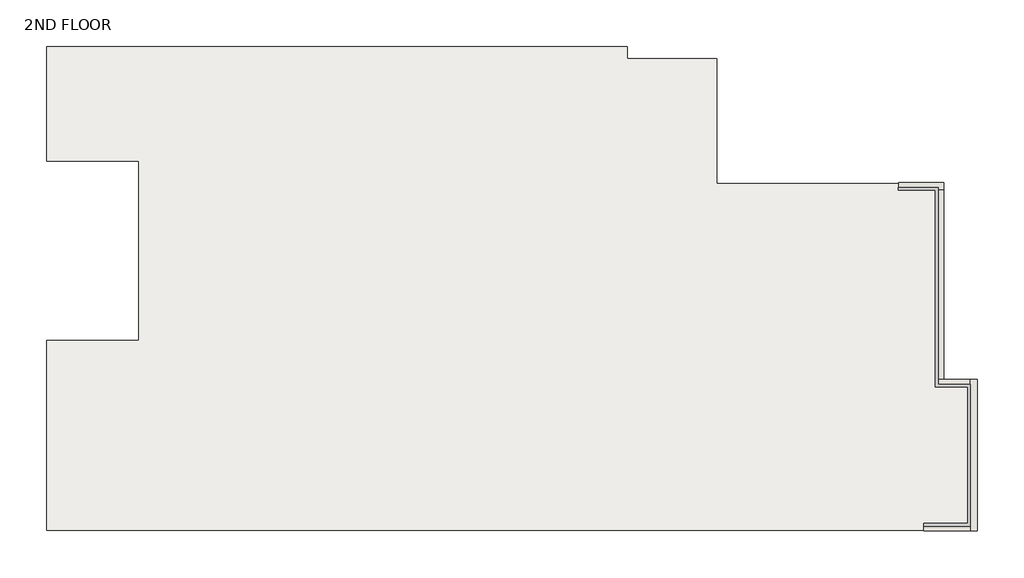
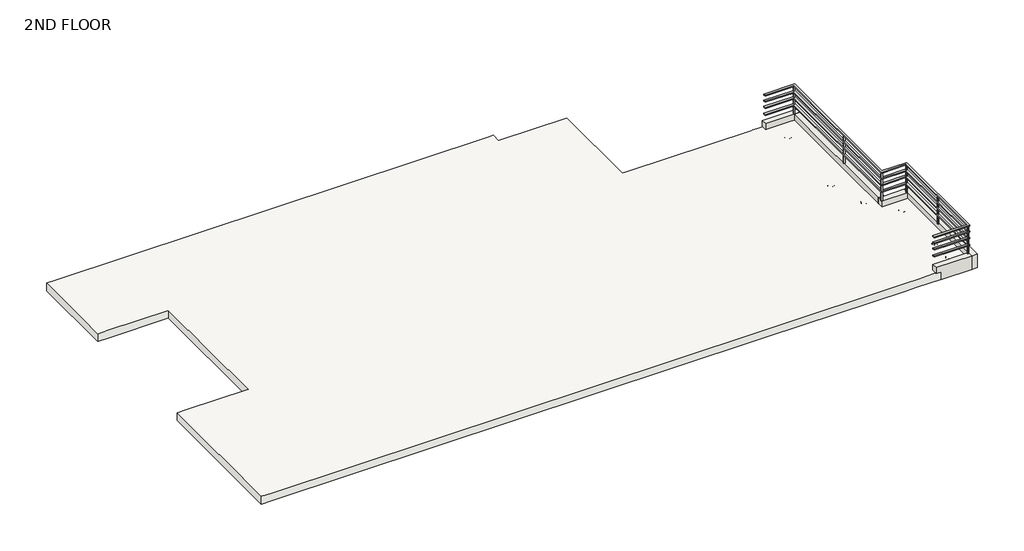
# One storey: 6 geographic elements, 5 proxies, 5 walls, 1 slab.
"""IFC4 building model written with IfcOpenShell, lengths in millimetres."""

import ifcopenshell
import ifcopenshell.guid

model = None  # the IFC model being written
_history = None  # IfcOwnerHistory: only IFC2X3 demands one
_inside = {}  # id of a spatial element -> (the spatial element, [elements in it])
_under = {}  # id of a project, library or spatial element -> (it, [spatial elements below it])
_declared = {}  # id of a project -> (the project, [libraries it declares])
_typed = {}  # id of a type object -> (the type object, [elements of that type])
_made_of = {}  # id of a material, layer set ... -> (it, [elements and type objects made of it])


def new_model(schema):
    """Start an empty IFC model of exactly this schema.

    Asked for "IFC4X3", IfcOpenShell would pick the latest addendum, in which some entities
    have other attributes; the version numbers below select the first issue.
    IFC2X3 requires an IfcOwnerHistory on every rooted entity: one is made here for all.
    """
    global model, _history
    if schema == "IFC4X3":
        model = ifcopenshell.file(schema_version=(4, 3, 0, 0))
    else:
        model = ifcopenshell.file(schema=schema)
    _inside.clear()
    _under.clear()
    _declared.clear()
    _typed.clear()
    _made_of.clear()
    _history = None
    if model.schema == "IFC2X3":
        org = make("IfcOrganization", Name="unknown")
        user = make(
            "IfcPersonAndOrganization",
            ThePerson=make("IfcPerson", FamilyName="unknown"),
            TheOrganization=org,
        )
        app = make(
            "IfcApplication",
            ApplicationDeveloper=org,
            Version="unknown",
            ApplicationFullName="unknown",
            ApplicationIdentifier="unknown",
        )
        _history = make(
            "IfcOwnerHistory",
            OwningUser=user,
            OwningApplication=app,
            ChangeAction="ADDED",
            CreationDate=0,
        )
    return model


def make(cls, **values):
    """One entity of the class cls with the attributes given. An attribute that is None is left unset."""
    return model.create_entity(
        cls, **{name: value for name, value in values.items() if value is not None}
    )


def rooted(cls, **values):
    """An entity with a GlobalId (a new one), such as an element, a storey or a relation."""
    return make(cls, GlobalId=ifcopenshell.guid.new(), OwnerHistory=_history, **values)


def si_unit(unit_type, name, prefix=None):
    """IfcSIUnit, for example si_unit("LENGTHUNIT", "METRE", prefix="MILLI")."""
    return make("IfcSIUnit", UnitType=unit_type, Prefix=prefix, Name=name)


def assignment(units):
    """IfcUnitAssignment: the units of a project."""
    return None if units is None else make("IfcUnitAssignment", Units=units)


def point(xyz):
    """IfcCartesianPoint."""
    return None if xyz is None else make("IfcCartesianPoint", Coordinates=xyz)


def direction(xyz):
    """IfcDirection."""
    return None if xyz is None else make("IfcDirection", DirectionRatios=xyz)


def frame(location, z_axis=None, x_axis=None):
    """IfcAxis2Placement3D, a coordinate frame: its origin and axes. An axis left out is left unset."""
    return make(
        "IfcAxis2Placement3D",
        Location=point(location),
        Axis=direction(z_axis),
        RefDirection=direction(x_axis),
    )


def origin():
    """The frame at (0, 0, 0) with its axes left unset."""
    return frame((0.0, 0.0, 0.0))


def place(relative_to, where):
    """IfcLocalPlacement: puts the frame where relative to a parent placement (None: the world)."""
    return make(
        "IfcLocalPlacement", PlacementRelTo=relative_to, RelativePlacement=where
    )


def context(
    kind, dimensions, precision=None, world=None, true_north=None, identifier=None
):
    """IfcGeometricRepresentationContext, for example the 3D "Model" context."""
    return make(
        "IfcGeometricRepresentationContext",
        ContextIdentifier=identifier,
        ContextType=kind,
        CoordinateSpaceDimension=dimensions,
        Precision=precision,
        WorldCoordinateSystem=world,
        TrueNorth=true_north,
    )


def project(units=None, contexts=None):
    """IfcProject with its units and contexts."""
    return rooted(
        "IfcProject",
        Name="project",
        RepresentationContexts=contexts,
        UnitsInContext=assignment(units),
    )


def spatial(cls, under=None, at=None, **own):
    """A site, building, storey or space (cls), placed at a placement, below another one or the project."""
    s = rooted(cls, ObjectPlacement=at, **own)
    if under is not None:
        _under.setdefault(under.id(), (under, []))[1].append(s)
    return s


def polyline(points):
    """IfcPolyline through the points."""
    return make("IfcPolyline", Points=[point(p) for p in points])


def outline(outer, holes=None, kind="AREA"):
    """IfcArbitraryClosedProfileDef: a profile drawn as a closed curve; with holes, ...WithVoids."""
    if holes is None:
        return make("IfcArbitraryClosedProfileDef", ProfileType=kind, OuterCurve=outer)
    return make(
        "IfcArbitraryProfileDefWithVoids",
        ProfileType=kind,
        OuterCurve=outer,
        InnerCurves=holes,
    )


def extrude(swept, where, along, depth):
    """IfcExtrudedAreaSolid: the profile swept, set in the frame where, extruded along a direction by depth."""
    return make(
        "IfcExtrudedAreaSolid",
        SweptArea=swept,
        Position=where,
        ExtrudedDirection=direction(along),
        Depth=depth,
    )


def faces_of(points, faces, orient=None, outer=None):
    """IfcFace entities. A face is a list of loops; a loop is a list of indices into points, from 0.

    orient and outer hold one flag for each loop. By default every Orientation is true, the
    first loop of a face is its IfcFaceOuterBound and the others are IfcFaceBound.
    """
    made = []
    for i, loops in enumerate(faces):
        bounds = []
        for j, loop in enumerate(loops):
            is_outer = j == 0 if outer is None else outer[i][j]
            bounds.append(
                make(
                    "IfcFaceOuterBound" if is_outer else "IfcFaceBound",
                    Bound=make("IfcPolyLoop", Polygon=[points[k] for k in loop]),
                    Orientation=True if orient is None else orient[i][j],
                )
            )
        made.append(make("IfcFace", Bounds=bounds))
    return made


def faceted_brep(points, faces, orient=None, outer=None, voids=None):
    """IfcFacetedBrep: a solid bounded by flat faces; with voids (closed shells), ...WithVoids."""
    shared = [point(p) for p in points]
    hull = make("IfcClosedShell", CfsFaces=faces_of(shared, faces, orient, outer))
    if voids is None:
        return make("IfcFacetedBrep", Outer=hull)
    return make(
        "IfcFacetedBrepWithVoids",
        Outer=hull,
        Voids=[
            make(cls, CfsFaces=faces_of(shared, fs, o, b)) for cls, fs, o, b in voids
        ],
    )


def shape(context_of_items, identifier, shape_type, items):
    """IfcShapeRepresentation: the items that make up one representation, for example the "Body"."""
    return make(
        "IfcShapeRepresentation",
        ContextOfItems=context_of_items,
        RepresentationIdentifier=identifier,
        RepresentationType=shape_type,
        Items=items,
    )


def source(mapping_origin, context_of_items, identifier, shape_type, items):
    """IfcRepresentationMap: a shape defined once, which mapped items show again and again."""
    return make(
        "IfcRepresentationMap",
        MappingOrigin=mapping_origin,
        MappedRepresentation=shape(context_of_items, identifier, shape_type, items),
    )


def transform(
    local_origin,
    x_axis=None,
    y_axis=None,
    z_axis=None,
    scale=None,
    scale2=None,
    scale3=None,
    uniform=True,
):
    """IfcCartesianTransformationOperator3D, or its non-uniform kind. x_axis, y_axis, z_axis: its Axis1, 2, 3."""
    if uniform:
        return make(
            "IfcCartesianTransformationOperator3D",
            Axis1=direction(x_axis),
            Axis2=direction(y_axis),
            LocalOrigin=point(local_origin),
            Scale=scale,
            Axis3=direction(z_axis),
        )
    return make(
        "IfcCartesianTransformationOperator3DnonUniform",
        Axis1=direction(x_axis),
        Axis2=direction(y_axis),
        LocalOrigin=point(local_origin),
        Scale=scale,
        Axis3=direction(z_axis),
        Scale2=scale2,
        Scale3=scale3,
    )


def mapped(mapping_source, mapping_target):
    """IfcMappedItem: shows the shape of a source again, moved by a transform."""
    return make(
        "IfcMappedItem", MappingSource=mapping_source, MappingTarget=mapping_target
    )


def made_of(thing, what):
    """Note that an element or type object is made of a material, layer set ...; save() writes the relation."""
    if what is not None:
        _made_of.setdefault(what.id(), (what, []))[1].append(thing)
    return thing


def element(
    cls,
    number,
    at=None,
    inside=None,
    cuts=None,
    type_object=None,
    material=None,
    context=None,
    identifier="Body",
    shape_type=None,
    held_by="IfcProductDefinitionShape",
    body=None,
    shapes=None,
    **own,
):
    """One element of the class cls, such as IfcWall. Its Tag is "e" and its number.

    at: its placement. inside: the storey or other place that contains it. cuts: it is an
    opening in that element (IfcRelVoidsElement). A single representation is given by context,
    identifier, shape_type and body (its items); several are given by shapes. held_by: the class
    of the entity that holds the representations. save() writes the other relations.
    """
    e = rooted(cls, Tag="e%d" % number, ObjectPlacement=at, **own)
    if body is not None:
        shapes = [shape(context, identifier, shape_type, body)]
    if shapes is not None:
        e.Representation = make(held_by, Representations=shapes)
    if inside is not None:
        _inside.setdefault(inside.id(), (inside, []))[1].append(e)
    if cuts is not None:
        rooted(
            "IfcRelVoidsElement", RelatingBuildingElement=cuts, RelatedOpeningElement=e
        )
    if type_object is not None:
        _typed.setdefault(type_object.id(), (type_object, []))[1].append(e)
    return made_of(e, material)


def aggregate(whole, parts):
    """IfcRelAggregates: a whole, such as a stair, and the parts it consists of."""
    return rooted("IfcRelAggregates", RelatingObject=whole, RelatedObjects=parts)


def save(model, path):
    """Write the relations noted so far, then the file.

    IfcRelAggregates (storeys below a building ...), IfcRelContainedInSpatialStructure (elements
    in a storey), IfcRelDefinesByType, IfcRelAssociatesMaterial and IfcRelDeclares: one each for
    every whole, place, type object, material and project.
    """
    for whole, parts in _under.values():
        aggregate(whole, parts)
    for where, things in _inside.values():
        rooted(
            "IfcRelContainedInSpatialStructure",
            RelatedElements=things,
            RelatingStructure=where,
        )
    for kind, things in _typed.values():
        rooted("IfcRelDefinesByType", RelatedObjects=things, RelatingType=kind)
    for what, things in _made_of.values():
        rooted("IfcRelAssociatesMaterial", RelatedObjects=things, RelatingMaterial=what)
    for by, libraries in _declared.values():
        rooted("IfcRelDeclares", RelatingContext=by, RelatedDefinitions=libraries)
    model.write(path)


def generic_models_1_generic_models_1_90de948b(model_context):
    return source(origin(), model_context, "Body", "SweptSolid", [
        extrude(outline(polyline([(17437.9879668, -9053.7860729), (17407.9879668, -9053.7860729), (17407.9879668, -9028.7860729), (17437.9879668, -9028.7860729), (17437.9879668, -9053.7860729)])), frame((0.0, 0.0, 6858.0), z_axis=(0.0, 0.0, 1.0), x_axis=(1.0, 0.0, 0.0)), (0.0, 0.0, 1.0), 722.1629366),
        extrude(outline(polyline([(17437.9879668, -7778.7860729), (17407.9879668, -7778.7860729), (17407.9879668, -7753.7860729), (17437.9879668, -7753.7860729), (17437.9879668, -7778.7860729)])), frame((0.0, 0.0, 6858.0), z_axis=(0.0, 0.0, 1.0), x_axis=(1.0, 0.0, 0.0)), (0.0, 0.0, 1.0), 722.1629366),
        extrude(outline(polyline([(17437.9879668, -6433.7860729), (17407.9879668, -6433.7860729), (17407.9879668, -6408.7860729), (17437.9879668, -6408.7860729), (17437.9879668, -6433.7860729)])), frame((0.0, 0.0, 6858.0), z_axis=(0.0, 0.0, 1.0), x_axis=(1.0, 0.0, 0.0)), (0.0, 0.0, 1.0), 722.1629366),
        extrude(outline(polyline([(16832.9879668, -6433.7860729), (16802.9879668, -6433.7860729), (16802.9879668, -6408.7860729), (16832.9879668, -6408.7860729), (16832.9879668, -6433.7860729)])), frame((0.0, 0.0, 6858.0), z_axis=(0.0, 0.0, 1.0), x_axis=(1.0, 0.0, 0.0)), (0.0, 0.0, 1.0), 722.1629366),
        extrude(outline(polyline([(16832.9879668, -4833.7860729), (16802.9879668, -4833.7860729), (16802.9879668, -4808.7860729), (16832.9879668, -4808.7860729), (16832.9879668, -4833.7860729)])), frame((0.0, 0.0, 6858.0), z_axis=(0.0, 0.0, 1.0), x_axis=(1.0, 0.0, 0.0)), (0.0, 0.0, 1.0), 722.1629366),
        extrude(outline(polyline([(16832.9879668, -2700.682032), (16802.9879668, -2700.682032), (16802.9879668, -2675.682032), (16832.9879668, -2675.682032), (16832.9879668, -2700.682032)])), frame((0.0, 0.0, 6858.0), z_axis=(0.0, 0.0, 1.0), x_axis=(1.0, 0.0, 0.0)), (0.0, 0.0, 1.0), 722.1629366),
    ])


def railing1_railing_f5fd7874(model_context):
    return source(origin(), model_context, "Body", "SweptSolid", [
        extrude(outline(polyline([(16573.5, -9069.3), (16573.5, -9019.3), (17401.9, -9019.3), (17401.9, -6436.6), (16791.7888874, -6436.6), (16791.7888874, -2715.5), (16090.9, -2715.5), (16090.9, -2665.5), (16841.7888874, -2665.5), (16841.7888874, -6386.6), (17451.9, -6386.6), (17451.9, -9069.3), (16573.5, -9069.3)])), frame((0.0, 0.0, 6858.0), z_axis=(0.0, 0.0, 1.0), x_axis=(1.0, 0.0, 0.0)), (0.0, 0.0, 1.0), 25.4370634),
    ])


def enscape_assetdefinition_ceiling_lamp_002_enscape_ece63965(model_context):
    return source(origin(), model_context, "Body", "Brep", [
        faceted_brep([(-78.1945959, 0.0, -170.0000018), (0.0, -78.1945959, -170.0000018), (-55.2917272, -55.2917272, -170.0000018), (-55.2917272, -55.2917272, 0.0), (55.2917272, -55.2917272, -170.0000018), (0.0, -78.1945959, 0.0), (-78.1945959, 0.0, 0.0), (0.0, 78.1945959, 0.0), (55.2917272, -55.2917272, 0.0), (78.1945959, 0.0, -170.0000018), (78.1945959, 0.0, 0.0), (55.2917272, 55.2917272, -170.0000018), (-55.2917272, 55.2917272, -170.0000018), (0.0, 78.1945959, -170.0000018), (55.2917272, 55.2917272, 0.0), (-55.2917272, 55.2917272, 0.0)], [[[0, 1, 2]], [[2, 1, 3]], [[1, 4, 5]], [[0, 4, 1]], [[3, 1, 5]], [[0, 2, 6]], [[6, 2, 3]], [[5, 6, 3]], [[5, 7, 6]], [[7, 5, 8]], [[5, 4, 8]], [[4, 9, 8]], [[0, 9, 4]], [[7, 8, 10]], [[8, 9, 10]], [[9, 11, 10]], [[9, 0, 12]], [[9, 12, 13]], [[9, 13, 11]], [[7, 10, 14]], [[10, 11, 14]], [[11, 13, 14]], [[13, 12, 7]], [[14, 13, 7]], [[6, 7, 15]], [[7, 12, 15]], [[15, 0, 6]], [[12, 0, 15]]]),
    ])


model = new_model("IFC4")

# Units and contexts
model_context = context("Model", 3, world=origin())
ifc_project = project(units=[si_unit("LENGTHUNIT", "METRE", prefix="MILLI")], contexts=[model_context])

# Site, building, storey
site = spatial("IfcSite", under=ifc_project)
building = spatial("IfcBuilding", under=site)
storey = spatial("IfcBuildingStorey", under=building, Name="2ND FLOOR", Elevation=6705.6)

# Proxies
placement = place(None, origin())
generic_models_1_generic_models_1_shape = generic_models_1_generic_models_1_90de948b(model_context)
element("IfcBuildingElementProxy", 1, Name="Generic Models 1 : Generic Models 1", ObjectType="Generic Models 1 : Generic Models 1", at=placement, inside=storey, context=model_context, shape_type="MappedRepresentation", body=[
    mapped(generic_models_1_generic_models_1_shape, transform((0.0, 0.0, 0.0), x_axis=(1.0, 0.0, 0.0), y_axis=(0.0, 1.0, 0.0), z_axis=(0.0, 0.0, 1.0))),
])
railing1_railing_shape = railing1_railing_f5fd7874(model_context)
element("IfcBuildingElementProxy", 2, Name="RAILING1 : RAILING", ObjectType="RAILING1 : RAILING", at=placement, inside=storey, context=model_context, shape_type="MappedRepresentation", body=[
    mapped(railing1_railing_shape, transform((0.0, 0.0, 220.0), x_axis=(1.0, 0.0, 0.0), y_axis=(0.0, 1.0, 0.0), z_axis=(0.0, 0.0, 1.0))),
])
element("IfcBuildingElementProxy", 3, Name="RAILING2 : RAILING", ObjectType="RAILING2 : RAILING", at=placement, inside=storey, context=model_context, shape_type="MappedRepresentation", body=[
    mapped(railing1_railing_shape, transform((0.0, 0.0, 400.0), x_axis=(1.0, 0.0, 0.0), y_axis=(0.0, 1.0, 0.0), z_axis=(0.0, 0.0, 1.0))),
])
element("IfcBuildingElementProxy", 4, Name="RAILING3 : RAILING", ObjectType="RAILING3 : RAILING", at=placement, inside=storey, context=model_context, shape_type="MappedRepresentation", body=[
    mapped(railing1_railing_shape, transform((0.0, 0.0, 560.0), x_axis=(1.0, 0.0, 0.0), y_axis=(0.0, 1.0, 0.0), z_axis=(0.0, 0.0, 1.0))),
])
element("IfcBuildingElementProxy", 5, Name="RAILING4 : RAILING", ObjectType="RAILING4 : RAILING", at=placement, inside=storey, context=model_context, shape_type="MappedRepresentation", body=[
    mapped(railing1_railing_shape, transform((0.0, 0.0, 722.1629366), x_axis=(1.0, 0.0, 0.0), y_axis=(0.0, 1.0, 0.0), z_axis=(0.0, 0.0, 1.0))),
])

# Geographic elements
enscape_assetdefinition_ceiling_lamp_002_enscape_shape = enscape_assetdefinition_ceiling_lamp_002_enscape_ece63965(model_context)
element("IfcGeographicElement", 6, ObjectType="Enscape AssetDefinition - Ceiling Lamp 002 : Enscape AssetDefinition - Ceiling Lamp 002", at=placement, inside=storey, context=model_context, shape_type="MappedRepresentation", body=[
    mapped(enscape_assetdefinition_ceiling_lamp_002_enscape_shape, transform((16376.6388874, -3190.1, 6705.6), x_axis=(1.0, 0.0, 0.0), y_axis=(0.0, 1.0, 0.0), z_axis=(0.0, 0.0, 1.0))),
])
element("IfcGeographicElement", 7, ObjectType="Enscape AssetDefinition - Ceiling Lamp 002 : Enscape AssetDefinition - Ceiling Lamp 002", at=placement, inside=storey, context=model_context, shape_type="MappedRepresentation", body=[
    mapped(enscape_assetdefinition_ceiling_lamp_002_enscape_shape, transform((16276.6388874, -5190.1, 6705.6), x_axis=(1.0, 0.0, 0.0), y_axis=(0.0, 1.0, 0.0), z_axis=(0.0, 0.0, 1.0))),
])
element("IfcGeographicElement", 8, ObjectType="Enscape AssetDefinition - Ceiling Lamp 002 : Enscape AssetDefinition - Ceiling Lamp 002", at=placement, inside=storey, context=model_context, shape_type="MappedRepresentation", body=[
    mapped(enscape_assetdefinition_ceiling_lamp_002_enscape_shape, transform((16576.6388874, -6090.1, 6705.6), x_axis=(1.0, 0.0, 0.0), y_axis=(0.0, 1.0, 0.0), z_axis=(0.0, 0.0, 1.0))),
])
element("IfcGeographicElement", 9, ObjectType="Enscape AssetDefinition - Ceiling Lamp 002 : Enscape AssetDefinition - Ceiling Lamp 002", at=placement, inside=storey, context=model_context, shape_type="MappedRepresentation", body=[
    mapped(enscape_assetdefinition_ceiling_lamp_002_enscape_shape, transform((17116.75, -6766.75, 6705.6), x_axis=(1.0, 0.0, 0.0), y_axis=(0.0, 1.0, 0.0), z_axis=(0.0, 0.0, 1.0))),
])
element("IfcGeographicElement", 10, ObjectType="Enscape AssetDefinition - Ceiling Lamp 002 : Enscape AssetDefinition - Ceiling Lamp 002", at=placement, inside=storey, context=model_context, shape_type="MappedRepresentation", body=[
    mapped(enscape_assetdefinition_ceiling_lamp_002_enscape_shape, transform((17116.75, -8166.75, 6705.6), x_axis=(1.0, 0.0, 0.0), y_axis=(0.0, 1.0, 0.0), z_axis=(0.0, 0.0, 1.0))),
])
element("IfcGeographicElement", 11, ObjectType="Enscape AssetDefinition - Ceiling Lamp 002 : Enscape AssetDefinition - Ceiling Lamp 002", at=placement, inside=storey, context=model_context, shape_type="MappedRepresentation", body=[
    mapped(enscape_assetdefinition_ceiling_lamp_002_enscape_shape, transform((17116.75, -8766.75, 6705.6), x_axis=(1.0, 0.0, 0.0), y_axis=(0.0, 1.0, 0.0), z_axis=(0.0, 0.0, 1.0))),
])

# Slab
element("IfcSlab", 12, ObjectType="PTS- FL- 8\" WITH FINISH", at=placement, inside=storey, context=model_context, shape_type="Brep", body=[
    faceted_brep([(0.0, -5562.6, 6502.4), (241.3, -5562.6, 6502.4), (1739.9, -5562.6, 6502.4), (1739.9, -2171.7, 6502.4), (241.3, -2171.7, 6502.4), (0.0, -2171.7, 6502.4), (0.0, 0.0, 6502.4), (241.3, 0.0, 6502.4), (10887.95, 0.0, 6502.4), (10972.8, 0.0, 6502.4), (10972.8, -228.6, 6502.4), (12656.8, -228.6, 6502.4), (12656.8, -2589.4, 6502.4), (12656.8, -2590.8, 6502.4), (12771.8, -2590.8, 6502.4), (15827.9, -2590.8, 6502.4), (15848.2, -2590.8, 6502.4), (16078.2, -2590.8, 6502.4), (16099.9, -2590.8, 6502.4), (16931.4888874, -2590.8, 6502.4), (16931.4888874, -6311.9, 6502.4), (17571.6, -6311.9, 6502.4), (17571.6, -9144.0, 6502.4), (16700.5, -9144.0, 6502.4), (16078.2, -9144.0, 6502.4), (15848.2, -9144.0, 6502.4), (12409.3, -9144.0, 6502.4), (12179.3, -9144.0, 6502.4), (241.3, -9144.0, 6502.4), (0.0, -9144.0, 6502.4), (0.0, -5562.6, 6705.6), (0.0, -9144.0, 6705.6), (241.3, -9144.0, 6705.6), (12179.3, -9144.0, 6705.6), (12409.3, -9144.0, 6705.6), (15848.2, -9144.0, 6705.6), (16078.2, -9144.0, 6705.6), (16573.5, -9144.0, 6705.6), (16700.5, -9144.0, 6705.6), (17571.6, -9144.0, 6705.6), (17571.6, -6311.9, 6705.6), (16931.4888874, -6311.9, 6705.6), (16931.4888874, -2590.8, 6705.6), (16099.9, -2590.8, 6705.6), (16078.2, -2590.8, 6705.6), (15848.2, -2590.8, 6705.6), (15827.9, -2590.8, 6705.6), (12771.8, -2590.8, 6705.6), (12656.8, -2590.8, 6705.6), (12656.8, -2589.4, 6705.6), (12656.8, -228.6, 6705.6), (10972.8, -228.6, 6705.6), (10972.8, 0.0, 6705.6), (10887.95, 0.0, 6705.6), (241.3, 0.0, 6705.6), (0.0, 0.0, 6705.6), (0.0, -2171.7, 6705.6), (241.3, -2171.7, 6705.6), (1739.9, -2171.7, 6705.6), (1739.9, -5562.6, 6705.6), (241.3, -5562.6, 6705.6)], [[[0, 1, 2, 3, 4, 5, 6, 7, 8, 9, 10, 11, 12, 13, 14, 15, 16, 17, 18, 19, 20, 21, 22, 23, 24, 25, 26, 27, 28, 29]], [[30, 31, 32, 33, 34, 35, 36, 37, 38, 39, 40, 41, 42, 43, 44, 45, 46, 47, 48, 49, 50, 51, 52, 53, 54, 55, 56, 57, 58, 59, 60]], [[9, 8, 7, 6, 55, 54, 53, 52]], [[20, 19, 42, 41]], [[29, 28, 27, 26, 25, 24, 23, 22, 39, 38, 37, 36, 35, 34, 33, 32, 31]], [[0, 29, 31, 30]], [[21, 20, 41, 40]], [[22, 21, 40, 39]], [[19, 18, 17, 16, 15, 14, 13, 48, 47, 46, 45, 44, 43, 42]], [[10, 9, 52, 51]], [[11, 10, 51, 50]], [[13, 12, 11, 50, 49, 48]], [[2, 1, 0, 30, 60, 59]], [[3, 2, 59, 58]], [[5, 4, 3, 58, 57, 56]], [[6, 5, 56, 55]]]),
])

# Walls
element("IfcWall", 13, ObjectType="PTS- BR- 4.5\"", at=placement, inside=storey, context=model_context, shape_type="Brep", body=[
    faceted_brep([(17586.6, -9161.3, 6502.4), (17586.6, -6296.9, 6502.4), (17586.6, -6296.9, 6858.0), (17586.6, -9161.3, 6858.0), (17446.9, -9161.3, 6502.4), (17446.9, -9161.3, 6858.0), (17446.9, -9021.6, 6858.0), (17446.9, -6436.6, 6858.0), (17446.9, -6296.9, 6858.0), (17446.9, -6296.9, 6502.4), (17446.9, -6436.6, 6502.4), (17446.9, -9021.6, 6502.4)], [[[0, 1, 2, 3]], [[4, 5, 6, 7, 8, 9, 10, 11]], [[1, 0, 4, 11, 10, 9]], [[3, 2, 8, 7, 6, 5]], [[0, 3, 5, 4]], [[2, 1, 9, 8]]]),
])
element("IfcWall", 14, ObjectType="PTS- BR- 4.5\"", at=placement, inside=storey, context=model_context, shape_type="Brep", body=[
    faceted_brep([(16700.5, -9161.3, 6502.4), (17446.9, -9161.3, 6502.4), (17446.9, -9161.3, 6858.0), (16573.5, -9161.3, 6858.0), (16573.5, -9161.3, 6705.6), (16700.5, -9161.3, 6705.6), (16700.5, -9021.6, 6502.4), (16700.5, -9021.6, 6705.6), (16573.5, -9021.6, 6705.6), (16573.5, -9021.6, 6858.0), (17446.9, -9021.6, 6858.0), (17446.9, -9021.6, 6502.4), (16573.5, -9144.0, 6705.6), (16573.5, -9159.0, 6705.6), (16700.5, -9144.0, 6705.6), (16700.5, -9159.0, 6705.6)], [[[0, 1, 2, 3, 4, 5]], [[6, 7, 8, 9, 10, 11]], [[1, 0, 6, 11]], [[3, 2, 10, 9]], [[2, 1, 11, 10]], [[4, 3, 9, 8, 12, 13]], [[4, 13, 12, 8, 7, 14, 15, 5]], [[0, 5, 15, 14, 7, 6]]]),
])
element("IfcWall", 15, ObjectType="PTS- BR- 4.5\"", at=placement, inside=storey, context=model_context, shape_type="Brep", body=[
    faceted_brep([(17446.9, -6296.9, 6502.4), (16946.4888874, -6296.9, 6502.4), (16806.7888874, -6296.9, 6502.4), (16806.7888874, -6296.9, 6858.0), (16946.4888874, -6296.9, 6858.0), (17446.9, -6296.9, 6858.0), (17446.9, -6436.6, 6502.4), (17446.9, -6436.6, 6858.0), (16806.7888874, -6436.6, 6858.0), (16806.7888874, -6436.6, 6502.4)], [[[0, 1, 2, 3, 4, 5]], [[6, 7, 8, 9]], [[2, 1, 0, 6, 9]], [[5, 4, 3, 8, 7]], [[3, 2, 9, 8]], [[0, 5, 7, 6]]]),
])
element("IfcWall", 16, ObjectType="PTS- BR- 4.5\"", at=placement, inside=storey, context=model_context, shape_type="Brep", body=[
    faceted_brep([(16099.9, -2715.5, 6858.0), (16099.9, -2715.5, 6502.4), (16806.7888874, -2715.5, 6502.4), (16946.4888874, -2715.5, 6502.4), (16946.4888874, -2715.5, 6858.0), (16806.7888874, -2715.5, 6858.0), (16099.9, -2575.8, 6502.4), (16099.9, -2575.8, 6858.0), (16946.4888874, -2575.8, 6858.0), (16946.4888874, -2575.8, 6502.4)], [[[0, 1, 2, 3, 4, 5]], [[6, 7, 8, 9]], [[3, 2, 1, 6, 9]], [[0, 5, 4, 8, 7]], [[4, 3, 9, 8]], [[0, 7, 6, 1]]]),
])
element("IfcWall", 17, ObjectType="PTS- BR- 4.5\"", at=placement, inside=storey, context=model_context, shape_type="SweptSolid", body=[
    extrude(outline(polyline([(16806.7888874, -6296.9), (16806.7888874, -2715.5), (16946.4888874, -2715.5), (16946.4888874, -6296.9), (16806.7888874, -6296.9)])), frame((0.0, 0.0, 6502.4), z_axis=(0.0, 0.0, 1.0), x_axis=(1.0, 0.0, 0.0)), (0.0, 0.0, 1.0), 355.6),
])

save(model, "model.ifc")

# Revit data of these elements
# Project information
#   Building Name = "RES. TYPE"
#   Project Issue Date = "11-06-2022"
#   Project Status = "Project Status"
#   Client Name = "AJAY KUMAR"
#   Project Address = "Enter address here"
#   Project Name = "Project Name"
#   Project Number = "PTS-132-RD-NNL-1"
# Grids (mm)
#   "1": line (-1730.266, -9029.7) -> (28901.358, -9029.7)
#   "2": line (-1730.266, -5505.45) -> (28901.358, -5505.45)
#   "3": line (-1730.266, -3943.35) -> (28901.358, -3943.35)
#   "4": line (-1730.266, -2705.1) -> (28901.358, -2705.1)
#   "5": line (-1730.266, -114.3) -> (28901.358, -114.3)
#   "A": line (114.3, -10604.021) -> (114.3, -114.3)
#   "B": line (1866.9, -10604.021) -> (1866.9, -114.3)
#   "C": line (6305.55, -10604.021) -> (6305.55, -114.3)
#   "D": line (10902.95, -10604.021) -> (10902.95, -114.3)
#   "E": line (15963.9, -10604.021) -> (15963.9, -114.3)
# Type "Enscape AssetDefinition - Ceiling Lamp 002 : Enscape AssetDefinition - Ceiling Lamp 002"
#   EnscapeAssetSource = "REMOTE"
#   EnscapeAssetId = "d2986385-ef04-40b6-b069-b70673c39d02"
#   EnscapeNativeAssetHeight = 0 mm
#   Height = 0
#   Default Elevation = 0
# Type "PTS- FL- 8\" WITH FINISH"
#   Assembly Code = "B1010"
#   Function = 0
#   Layers, outside or top first: 50.8 mm "Render Material 255-255-0" (function 1); 152.4 mm "Concrete, Cast-in-Place gray" (function 1)
# Type "PTS- BR- 4.5\""
#   Assembly Code = "B2010"
#   Layers, outside or top first: 12.7 mm "PLASTER MAT" (function 4); 114.3 mm "Brick, Common" (function 1); 12.7 mm "PLASTER MAT" (function 4)
# Element 1 (IfcBuildingElementProxy, "Generic Models 1 : Generic Models 1")
#   Phase Created = New Construction
#   Materials on its faces: "METAL TEXTURE"
# Element 2 (IfcBuildingElementProxy, "RAILING1 : RAILING")
#   Phase Created = New Construction
#   Materials on its faces: "METAL TEXTURE"
# Element 3 (IfcBuildingElementProxy, "RAILING2 : RAILING")
#   Phase Created = New Construction
#   Materials on its faces: "METAL TEXTURE"
# Element 4 (IfcBuildingElementProxy, "RAILING3 : RAILING")
#   Phase Created = New Construction
#   Materials on its faces: "METAL TEXTURE"
# Element 5 (IfcBuildingElementProxy, "RAILING4 : RAILING")
#   Phase Created = New Construction
#   Materials on its faces: "METAL TEXTURE"
# Elements 6, 7, 8, 9, 10, 11 (IfcGeographicElement, "Enscape AssetDefinition - Ceiling Lamp 002 : Enscape AssetDefinition - Ceiling Lamp 002")
#   Phase Created = New Construction
# Element 12 (IfcSlab, "PTS- FL- 8\" WITH FINISH")
#   built-in parameter 1001955 = 1.5708 (stored number, unit not read)
#   Height Offset From Level = 0 mm
#   built-in parameter 1001954 = 1
#   Phase Created = New Construction
#   Materials on its faces: "Concrete, Cast-in-Place gray", "Render Material 255-255-0"
# Element 13 (IfcWall, "PTS- BR- 4.5\"")
#   built-in parameter 1001111 = -203.2 mm
#   Top Offset = 0 mm
#   Base Offset = -203.2 mm
#   Unconnected Height = 355.6 mm
#   wall height = 355.6 mm
#   Phase Created = New Construction
#   Base Constraint = 2ND FLOOR
#   Materials on its faces: "P6", "PLASTER MAT", "Default Wall"
# Element 14 (IfcWall, "PTS- BR- 4.5\"")
#   built-in parameter 1001111 = -203.2 mm
#   Top Offset = 0 mm
#   Base Offset = -203.2 mm
#   Unconnected Height = 355.6 mm
#   wall height = 355.6 mm
#   Phase Created = New Construction
#   Base Constraint = 2ND FLOOR
#   Materials on its faces: "Default Wall", "PLASTER MAT"
# Elements 15, 16, 17 (IfcWall, "PTS- BR- 4.5\"")
#   built-in parameter 1001111 = -203.2 mm
#   Top Offset = 0 mm
#   Base Offset = -203.2 mm
#   Unconnected Height = 355.6 mm
#   wall height = 355.6 mm
#   Phase Created = New Construction
#   Base Constraint = 2ND FLOOR
#   Materials on its faces: "Default Wall", "PLASTER MAT", "P6"
# Materials
#   "Render Material 255-255-0": class "Unassigned", colour RGB 255 255 0, transparency 0, Comments = "Rendering appearance not upgraded "
#   "Concrete, Cast-in-Place gray": class "Concrete", colour RGB 192 192 192, transparency 0, Description = "Cast-in-place concrete", Cost = 0
#   "PLASTER MAT": class "Generic", colour RGB 120 120 120, transparency 0, Cost = 0
#   "Brick, Common": class "Masonry", colour RGB 192 192 192, transparency 0, Description = "Common brick", Cost = 0
#   "METAL TEXTURE": class "Generic", colour RGB 120 120 120, transparency 0, Cost = 0
#   "P6": class "Generic", colour RGB 120 120 120, transparency 0, Cost = 0
#   "Default Wall": class "Miscellaneous", colour RGB 128 128 128, transparency 0, Cost = 0
